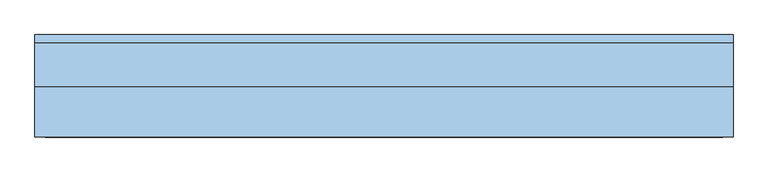
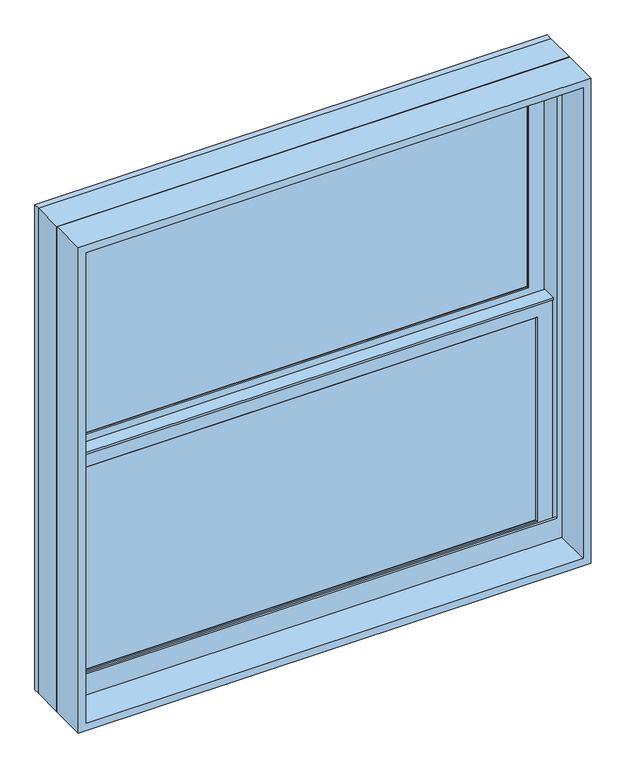
"""IFC4 building model written with IfcOpenShell, lengths in millimetres: window geometry, Window-Double_Hung-Marvin-Essential : ESDH3636."""

from ifc_helpers import new_model, si_unit, frame, origin, place, context, project, spatial, polyline, outline, extrude, faceted_brep, source, transform, mapped, element, save


def window_6cd664cb(model_context):
    return source(origin(), model_context, "Body", "SolidModel", [
        extrude(outline(polyline([(166.1583333, 20.6375), (166.1583333, 15.875), (147.1083333, 15.875), (147.1083333, 20.6375), (166.1583333, 20.6375)])), frame((0.0, 0.0, 1441.45), z_axis=(0.0, 0.0, 1.0), x_axis=(1.0, 0.0, 0.0)), (0.0, 0.0, 1.0), 450.85),
        extrude(outline(polyline([(-147.1083333, 20.6375), (-147.1083333, 15.875), (-166.1583333, 15.875), (-166.1583333, 20.6375), (-147.1083333, 20.6375)])), frame((0.0, 0.0, 1441.45), z_axis=(0.0, 0.0, 1.0), x_axis=(1.0, 0.0, 0.0)), (0.0, 0.0, 1.0), 450.85),
        extrude(outline(polyline([(469.9, 20.6375), (469.9, 15.875), (-469.9, 15.875), (-469.9, 20.6375), (469.9, 20.6375)])), frame((0.0, 0.0, 1657.35), z_axis=(0.0, 0.0, 1.0), x_axis=(1.0, 0.0, 0.0)), (0.0, 0.0, 1.0), 19.05),
        extrude(outline(polyline([(-166.1583333, 46.83125), (-166.1583333, 51.59375), (-147.1083333, 51.59375), (-147.1083333, 46.83125), (-166.1583333, 46.83125)])), frame((0.0, 0.0, 1930.4), z_axis=(0.0, 0.0, 1.0), x_axis=(1.0, 0.0, 0.0)), (0.0, 0.0, 1.0), 450.85),
        extrude(outline(polyline([(147.1083333, 46.83125), (147.1083333, 51.59375), (166.1583333, 51.59375), (166.1583333, 46.83125), (147.1083333, 46.83125)])), frame((0.0, 0.0, 1930.4), z_axis=(0.0, 0.0, 1.0), x_axis=(1.0, 0.0, 0.0)), (0.0, 0.0, 1.0), 450.85),
        extrude(outline(polyline([(-469.9, 46.83125), (-469.9, 51.59375), (469.9, 51.59375), (469.9, 46.83125), (-469.9, 46.83125)])), frame((0.0, 0.0, 2146.3), z_axis=(0.0, 0.0, 1.0), x_axis=(1.0, 0.0, 0.0)), (0.0, 0.0, 1.0), 19.05),
        extrude(outline(polyline([(166.1583333, 20.6375), (147.1083333, 20.6375), (147.1083333, 25.4), (166.1583333, 25.4), (166.1583333, 20.6375)])), frame((0.0, 0.0, 1441.45), z_axis=(0.0, 0.0, 1.0), x_axis=(1.0, 0.0, 0.0)), (0.0, 0.0, 1.0), 450.85),
        extrude(outline(polyline([(-147.1083333, 20.6375), (-166.1583333, 20.6375), (-166.1583333, 25.4), (-147.1083333, 25.4), (-147.1083333, 20.6375)])), frame((0.0, 0.0, 1441.45), z_axis=(0.0, 0.0, 1.0), x_axis=(1.0, 0.0, 0.0)), (0.0, 0.0, 1.0), 450.85),
        extrude(outline(polyline([(469.9, 20.6375), (-469.9, 20.6375), (-469.9, 25.4), (469.9, 25.4), (469.9, 20.6375)])), frame((0.0, 0.0, 1657.35), z_axis=(0.0, 0.0, 1.0), x_axis=(1.0, 0.0, 0.0)), (0.0, 0.0, 1.0), 19.05),
        extrude(outline(polyline([(-166.1583333, 56.35625), (-147.1083333, 56.35625), (-147.1083333, 51.59375), (-166.1583333, 51.59375), (-166.1583333, 56.35625)])), frame((0.0, 0.0, 1930.4), z_axis=(0.0, 0.0, 1.0), x_axis=(1.0, 0.0, 0.0)), (0.0, 0.0, 1.0), 450.85),
        extrude(outline(polyline([(147.1083333, 56.35625), (166.1583333, 56.35625), (166.1583333, 51.59375), (147.1083333, 51.59375), (147.1083333, 56.35625)])), frame((0.0, 0.0, 1930.4), z_axis=(0.0, 0.0, 1.0), x_axis=(1.0, 0.0, 0.0)), (0.0, 0.0, 1.0), 450.85),
        extrude(outline(polyline([(-469.9, 56.35625), (469.9, 56.35625), (469.9, 51.59375), (-469.9, 51.59375), (-469.9, 56.35625)])), frame((0.0, 0.0, 2146.3), z_axis=(0.0, 0.0, 1.0), x_axis=(1.0, 0.0, 0.0)), (0.0, 0.0, 1.0), 19.05),
        faceted_brep([(-496.8875, 5.6780605, 1922.3351748), (-496.8875, 5.6780605, 1917.7), (496.8875, 5.6780605, 1917.7), (496.8875, 5.6780605, 1922.3351748), (-496.8875, 34.8118605, 1922.3351748), (496.8875, 34.8118605, 1922.3351748), (496.8875, 34.8118605, 1917.7), (-496.8875, 34.8118605, 1917.7), (-496.8875, 30.1625, 1917.7), (-496.8875, 30.1625, 1414.4625), (-496.8875, 8.9241104, 1414.4625), (-496.8875, 8.9241104, 1917.7), (496.8875, 8.9241104, 1917.7), (496.8875, 30.1625, 1917.7), (496.8875, 8.9241104, 1414.4625), (496.8875, 30.1625, 1414.4625), (-481.0034752, 11.90625, 1903.4034752), (-481.0034752, 30.1625, 1903.4034752), (481.0034752, 30.1625, 1903.4034752), (481.0034752, 11.90625, 1903.4034752), (-464.34375, 10.4662439, 1886.74375), (-464.34375, 11.90625, 1886.74375), (464.34375, 11.90625, 1886.74375), (464.34375, 10.4662439, 1886.74375), (465.8858834, 8.9241104, 1888.2858834), (-465.8858834, 8.9241104, 1888.2858834), (481.0034752, 30.1625, 1430.3465248), (481.0034752, 11.90625, 1430.3465248), (464.34375, 11.90625, 1447.00625), (464.34375, 10.4662439, 1447.00625), (465.8858834, 8.9241104, 1445.4641166), (-481.0034752, 30.1625, 1430.3465248), (-481.0034752, 11.90625, 1430.3465248), (-464.34375, 11.90625, 1447.00625), (-464.34375, 10.4662439, 1447.00625), (-465.8858834, 8.9241104, 1445.4641166)], [[[0, 1, 2, 3]], [[4, 5, 6, 7]], [[1, 0, 4, 7, 8, 9, 10, 11]], [[2, 1, 11, 12]], [[7, 6, 13, 8]], [[3, 2, 12, 14, 15, 13, 6, 5]], [[0, 3, 5, 4]], [[16, 17, 18, 19]], [[20, 21, 22, 23]], [[20, 23, 24, 25]], [[19, 18, 26, 27]], [[23, 22, 28, 29]], [[24, 23, 29, 30]], [[27, 26, 31, 32]], [[29, 28, 33, 34]], [[30, 29, 34, 35]], [[15, 14, 10, 9]], [[15, 9, 8, 13], [18, 17, 31, 26]], [[17, 16, 32, 31]], [[16, 19, 27, 32], [22, 21, 33, 28]], [[21, 20, 34, 33]], [[20, 25, 35, 34]], [[10, 14, 12, 11], [25, 24, 30, 35]]]),
        extrude(outline(polyline([(38.5955581, 1903.4125), (33.5778968, 1903.4125), (33.5778968, 1905.0), (39.9405976, 1905.0), (39.9405976, 1903.4125), (61.515625, 1903.4125), (47.6307501, 1900.0975159), (38.5955581, 1900.0975159), (38.5955581, 1903.4125)])), frame((-496.8875, 0.0, 0.0), z_axis=(1.0, 0.0, 0.0), x_axis=(0.0, 1.0, 0.0)), (0.0, 0.0, 1.0), 993.775),
        faceted_brep([(527.05, 0.0, 1384.3), (527.05, 0.0, 2438.4), (-527.05, 0.0, 2438.4), (-527.05, 0.0, 1384.3), (500.85625, 0.0, 1445.41875), (-500.85625, 0.0, 1445.41875), (-500.85625, 0.0, 2412.20625), (500.85625, 0.0, 2412.20625), (500.85625, 3.96875, 1384.3), (-500.85625, 3.96875, 1384.3), (-500.85625, 3.96875, 1445.41875), (500.85625, 3.96875, 1445.41875), (-527.05, 65.6828125, 1384.3), (-500.85625, 65.6828125, 1384.3), (500.85625, 65.6828125, 1384.3), (527.05, 65.6828125, 1384.3), (-527.05, 65.6828125, 2438.4), (527.05, 65.6828125, 2438.4), (500.85625, 65.6828125, 2412.20625), (-500.85625, 65.6828125, 2412.20625)], [[[0, 1, 2, 3], [4, 5, 6, 7]], [[8, 9, 10, 11]], [[5, 4, 11, 10]], [[0, 3, 12, 13, 9, 8, 14, 15]], [[13, 12, 16, 17, 15, 14, 18, 19]], [[13, 19, 6, 5, 10, 9]], [[7, 6, 19, 18]], [[18, 14, 8, 11, 4, 7]], [[1, 0, 15, 17]], [[2, 1, 17, 16]], [[3, 2, 16, 12]]]),
        faceted_brep([(500.85625, 30.1625, 1911.35), (499.26875, 30.1625, 1911.35), (499.26875, 30.1625, 1408.6544613), (500.85625, 30.1625, 1408.6544613), (-499.26875, 30.1625, 1911.35), (-500.85625, 30.1625, 1911.35), (-500.85625, 30.1625, 1408.6544613), (-499.26875, 30.1625, 1408.6544613), (499.26875, 63.5, 1911.35), (500.85625, 63.5, 1911.35), (500.85625, 63.5, 1402.1743077), (499.26875, 63.5, 1402.1743077), (-500.85625, 63.5, 1911.35), (-499.26875, 63.5, 1911.35), (-499.26875, 63.5, 1402.1743077), (-500.85625, 63.5, 1402.1743077), (512.1108932, 3.96875, 1413.7460105), (512.1108932, 3.96875, 1384.3), (512.1108932, 65.6828125, 1384.3), (512.1108932, 65.6828125, 1401.750012), (-512.1108932, 3.96875, 1384.3), (-512.1108932, 3.96875, 1413.7460105), (-512.1108932, 65.6828125, 1401.750012), (-512.1108932, 65.6828125, 1384.3), (512.1108932, 78.58125, 1399.2428097), (-512.1108932, 78.58125, 1399.2428097), (-510.0971252, 68.2348864, 1401.2539391), (-492.13135, 68.2348864, 1401.2539391), (-492.13135, 65.6828125, 1401.750012), (492.13135, 65.6828125, 1401.750012), (492.13135, 68.2348864, 1401.2539391), (510.0971252, 68.2348864, 1401.2539391), (-527.05, 65.6828125, 1384.3), (-527.05, 78.5948249, 1384.3), (527.05, 78.5948249, 1384.3), (527.05, 65.6828125, 1384.3), (-527.05, 78.58125, 2438.4), (527.05, 78.58125, 2438.4), (512.1108932, 78.58125, 2423.4608932), (-512.1108932, 78.58125, 2423.4608932), (-527.05, 65.6828125, 2438.4), (-510.0971252, 68.2348864, 2421.4471252), (510.0971252, 68.2348864, 2421.4471252), (492.13135, 68.2348864, 2403.48135), (-492.13135, 68.2348864, 2403.48135), (-492.13135, 65.6828125, 2403.48135), (492.13135, 65.6828125, 2403.48135), (527.05, 65.6828125, 2438.4)], [[[0, 1, 2, 3]], [[4, 5, 6, 7]], [[8, 9, 10, 11]], [[12, 13, 14, 15]], [[1, 8, 11, 2]], [[9, 0, 3, 10]], [[1, 0, 9, 8]], [[5, 4, 13, 12]], [[5, 12, 15, 6]], [[13, 4, 7, 14]], [[16, 17, 18, 19]], [[20, 21, 22, 23]], [[24, 25, 26, 27, 28, 22, 21, 16, 19, 29, 30, 31], [3, 2, 11, 10], [7, 6, 15, 14]], [[17, 16, 21, 20]], [[17, 20, 23, 32, 33, 34, 35, 18]], [[34, 33, 36, 37], [25, 24, 38, 39]], [[33, 32, 40, 36]], [[39, 41, 26, 25]], [[41, 42, 31, 30, 43, 44, 27, 26]], [[44, 45, 28, 27]], [[40, 32, 23, 22, 28, 45, 46, 29, 19, 18, 35, 47]], [[36, 40, 47, 37]], [[39, 38, 42, 41]], [[44, 43, 46, 45]], [[34, 37, 47, 35]], [[42, 38, 24, 31]], [[46, 43, 30, 29]]]),
        extrude(outline(polyline([(477.04375, 11.90625), (-477.04375, 11.90625), (-477.04375, 15.08125), (477.04375, 15.08125), (477.04375, 11.90625)])), frame((0.0, 0.0, 1434.30625), z_axis=(0.0, 0.0, 1.0), x_axis=(1.0, 0.0, 0.0)), (0.0, 0.0, 1.0), 465.1375),
        extrude(outline(polyline([(477.04375, 42.8625), (-477.04375, 42.8625), (-477.04375, 46.0375), (477.04375, 46.0375), (477.04375, 42.8625)])), frame((0.0, 0.0, 1923.25625), z_axis=(0.0, 0.0, 1.0), x_axis=(1.0, 0.0, 0.0)), (0.0, 0.0, 1.0), 465.1375),
        faceted_brep([(-464.34375, 31.194477, 1886.74375), (-465.8858834, 32.7366104, 1888.2858834), (465.8858834, 32.7366104, 1888.2858834), (464.34375, 31.194477, 1886.74375), (-464.34375, 30.1625, 1886.74375), (464.34375, 30.1625, 1886.74375), (-496.8875, 32.7366104, 1919.2875), (-496.8875, 30.1625, 1919.2875), (496.8875, 30.1625, 1919.2875), (496.8875, 32.7366104, 1919.2875), (465.8858834, 32.7366104, 1445.4641166), (464.34375, 31.194477, 1447.00625), (464.34375, 30.1625, 1447.00625), (496.8875, 30.1625, 1414.4625), (496.8875, 32.7366104, 1414.4625), (-465.8858834, 32.7366104, 1445.4641166), (-464.34375, 31.194477, 1447.00625), (-464.34375, 30.1625, 1447.00625), (-496.8875, 30.1625, 1414.4625), (-496.8875, 32.7366104, 1414.4625)], [[[0, 1, 2, 3]], [[4, 0, 3, 5]], [[6, 7, 8, 9]], [[3, 2, 10, 11]], [[5, 3, 11, 12]], [[9, 8, 13, 14]], [[11, 10, 15, 16]], [[12, 11, 16, 17]], [[14, 13, 18, 19]], [[9, 14, 19, 6], [1, 15, 10, 2]], [[16, 15, 1, 0]], [[17, 16, 0, 4]], [[7, 18, 13, 8], [5, 12, 17, 4]], [[19, 18, 7, 6]]]),
        faceted_brep([(-481.0034752, 42.8625, 2392.3534752), (-481.0034752, 61.11875, 2392.3534752), (481.0034752, 61.11875, 2392.3534752), (481.0034752, 42.8625, 2392.3534752), (-464.34375, 41.4224939, 2375.69375), (-464.34375, 42.8625, 2375.69375), (464.34375, 42.8625, 2375.69375), (464.34375, 41.4224939, 2375.69375), (-465.8858834, 39.8803604, 2377.2358834), (465.8858834, 39.8803604, 2377.2358834), (-496.8875, 61.11875, 2408.2375), (-496.8875, 39.8803604, 2408.2375), (496.8875, 39.8803604, 2408.2375), (496.8875, 61.11875, 2408.2375), (481.0034752, 61.11875, 1919.2965248), (481.0034752, 42.8625, 1919.2965248), (464.34375, 42.8625, 1935.95625), (464.34375, 41.4224939, 1935.95625), (465.8858834, 39.8803604, 1934.4141166), (496.8875, 39.8803604, 1903.4125), (496.8875, 61.11875, 1903.4125), (-481.0034752, 61.11875, 1919.2965248), (-481.0034752, 42.8625, 1919.2965248), (-464.34375, 42.8625, 1935.95625), (-464.34375, 41.4224939, 1935.95625), (-465.8858834, 39.8803604, 1934.4141166), (-496.8875, 39.8803604, 1903.4125), (-496.8875, 61.11875, 1903.4125)], [[[0, 1, 2, 3]], [[4, 5, 6, 7]], [[8, 4, 7, 9]], [[10, 11, 12, 13]], [[3, 2, 14, 15]], [[7, 6, 16, 17]], [[9, 7, 17, 18]], [[13, 12, 19, 20]], [[15, 14, 21, 22]], [[17, 16, 23, 24]], [[18, 17, 24, 25]], [[20, 19, 26, 27]], [[13, 20, 27, 10], [1, 21, 14, 2]], [[22, 21, 1, 0]], [[3, 15, 22, 0], [5, 23, 16, 6]], [[24, 23, 5, 4]], [[25, 24, 4, 8]], [[11, 26, 19, 12], [9, 18, 25, 8]], [[27, 26, 11, 10]]]),
        faceted_brep([(-496.8875, 61.11875, 1903.4125), (-496.8875, 63.6928604, 1903.4125), (496.8875, 63.6928604, 1903.4125), (496.8875, 61.11875, 1903.4125), (-464.34375, 62.150727, 1935.95625), (-464.34375, 61.11875, 1935.95625), (464.34375, 61.11875, 1935.95625), (464.34375, 62.150727, 1935.95625), (-465.8858834, 63.6928604, 1934.4141166), (465.8858834, 63.6928604, 1934.4141166), (496.8875, 63.6928604, 2408.2375), (496.8875, 61.11875, 2408.2375), (464.34375, 61.11875, 2375.69375), (464.34375, 62.150727, 2375.69375), (465.8858834, 63.6928604, 2377.2358834), (-496.8875, 63.6928604, 2408.2375), (-496.8875, 61.11875, 2408.2375), (-464.34375, 61.11875, 2375.69375), (-464.34375, 62.150727, 2375.69375), (-465.8858834, 63.6928604, 2377.2358834)], [[[0, 1, 2, 3]], [[4, 5, 6, 7]], [[8, 4, 7, 9]], [[3, 2, 10, 11]], [[7, 6, 12, 13]], [[9, 7, 13, 14]], [[11, 10, 15, 16]], [[13, 12, 17, 18]], [[14, 13, 18, 19]], [[16, 15, 1, 0]], [[3, 11, 16, 0], [5, 17, 12, 6]], [[18, 17, 5, 4]], [[19, 18, 4, 8]], [[1, 15, 10, 2], [9, 14, 19, 8]]]),
        extrude(outline(polyline([(477.04375, 26.19375), (-477.04375, 26.19375), (-477.04375, 30.1625), (477.04375, 30.1625), (477.04375, 26.19375)])), frame((0.0, 0.0, 1434.30625), z_axis=(0.0, 0.0, 1.0), x_axis=(1.0, 0.0, 0.0)), (0.0, 0.0, 1.0), 465.1375),
        extrude(outline(polyline([(477.04375, 57.15), (-477.04375, 57.15), (-477.04375, 61.11875), (477.04375, 61.11875), (477.04375, 57.15)])), frame((0.0, 0.0, 1923.25625), z_axis=(0.0, 0.0, 1.0), x_axis=(1.0, 0.0, 0.0)), (0.0, 0.0, 1.0), 465.1375),
        extrude(outline(polyline([(2438.4, 527.05), (2438.4, -527.05), (1384.3, -527.05), (1384.3, 527.05), (2438.4, 527.05)]), holes=[polyline([(2422.525, 511.175), (1400.175, 511.175), (1400.175, -511.175), (2422.525, -511.175), (2422.525, 511.175)])]), frame((0.0, -76.2, 0.0), z_axis=(0.0, 1.0, 0.0), x_axis=(0.0, 0.0, 1.0)), (0.0, 0.0, 1.0), 75.40625),
    ])


if __name__ == "__main__":
    model = new_model("IFC4")
    model_context = context("Model", 3, world=origin())
    ifc_project = project(units=[si_unit("LENGTHUNIT", "METRE", prefix="MILLI")], contexts=[model_context])
    site = spatial("IfcSite", under=ifc_project)
    building = spatial("IfcBuilding", under=site)
    placement = place(None, origin())
    window_shape = window_6cd664cb(model_context)
    element("IfcWindow", 1, ObjectType="Window-Double_Hung-Marvin-Essential : ESDH3636", at=placement, inside=building, context=model_context, shape_type="MappedRepresentation", body=[
        mapped(window_shape, transform((0.0, 0.0, 0.0), x_axis=(1.0, 0.0, 0.0), y_axis=(0.0, 1.0, 0.0), z_axis=(0.0, 0.0, 1.0))),
    ])
    save(model, "model.ifc")

# Revit data of these elements
# Type "Window-Double_Hung-Marvin-Essential : ESDH3636"
#   Type Mark = "45"
#   Window Type = "Essential Double Hung"
#   Product data url = "https://bimobject.com/marvin-windows-and-doors/product/marvin-dhwau"
#   Product Guid = "c4a96547-874c-4385-91dc-a058adc19d98"
#   Frame = "All Ultrex"
#   Egress Window = "No"
#   URL = "www.marvin.com"
#   Model = "ESDH3636"
#   Manufacturer = "Marvin Windows and Doors"
#   Label Egress = ""
#   Glass Type = "IG Low E II with Argon"
#   Design Pressure = "DP50"
#   Description = "4242 DBHG"
#   Analytic Construction = "<None>"
#   Prairie Corner Width = 0' - 4"
#   Prairie Corner Height = 0' - 4"
#   Egress Width = 3' - 2 9/16"
#   Egress Height = 1' - 4 27/128"
#   Rough Width = 3' - 6"
#   Rough Height = 3' - 6"
#   Nominal Width = 3' - 6"
#   Nominal Height = 3' - 6"
#   Inset to Installation Flange [instance default] = 0' - 1"
#   Height = 3' - 5 1/2"
#   Egress Area = 4.34121 SF
#   Default Head Height = 8' - 0"
#   Width = 3' - 5 1/2"
#   Daylight Area = 8.7915 SF
#   DLO Width = 3' - 0 9/16"
#   DLO Height = 1' - 5 5/16"
#   Muntins Top Sash = yes
#   Lites Wide Top Sash = 3
#   Lites Wide Bottom Sash = 3
#   Lites High Top Sash = 2
#   Lites High Bottom Sash = 2
#   Lite Cut Prairie 9 = no
#   Lite Cut HV Grid = yes
#   Muntins Bottom Sash = yes
#   Label Visibility = no
#   Jamb Extension Visibility = yes
#   Edition number = 1
#   Interior Material = Ultrex-Marvin-Stonewhite
#   Glazing Material = Glass-Marvin-IG Low E II with Argon
#   Cladding Material = Ultrex-Marvin-Pebblegray
#   Wall Closure = (empty or 0)
#   Assembly Code = ""
# Element 1 (IfcWindow, "Window-Double_Hung-Marvin-Essential : ESDH3636")
#   Materials on its faces: "Ultrex-Marvin-Pebblegray", "Ultrex-Marvin-Stonewhite", "Glass-Marvin-IG Low E II with Argon"
# Materials
#   "Ultrex-Marvin-Stonewhite": class "Paint", colour RGB 250 251 245, transparency 0
#   "Glass-Marvin-IG Low E II with Argon": class "Glass", colour RGB 0 128 192, transparency 0.85
#   "Ultrex-Marvin-Pebblegray": class "Paint", colour RGB 189 185 173, transparency 0
